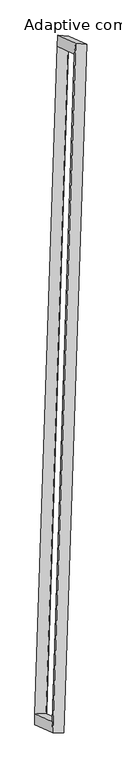
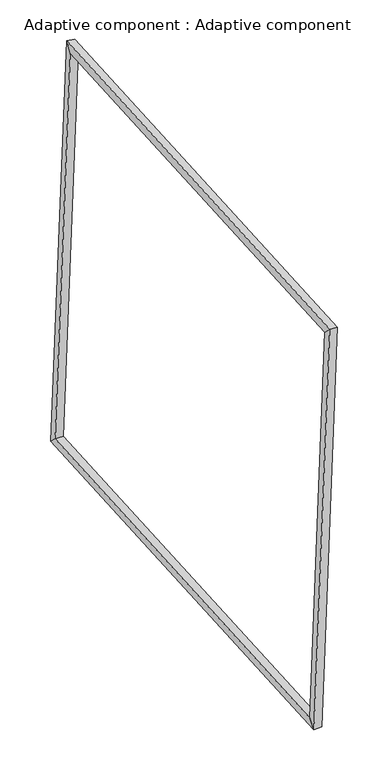
"""IFC4 building model written with IfcOpenShell, lengths in millimetres: proxy geometry, Adaptive component : Adaptive component."""

from ifc_helpers import new_model, si_unit, origin, place, context, project, spatial, faceted_brep, source, transform, mapped, element, save


def adaptive_component_adaptive_component_f8707263(model_context):
    return source(origin(), model_context, "Body", "Brep", [
        faceted_brep([(90.3369049, 1495.2326246, 3057.0965075), (154.9507537, 1489.5796526, 3051.5404015), (26.4269015, -2378.2634485, 3002.3473224), (-38.4243389, -2379.7546235, 3007.8125658), (97.9728871, 1559.0874571, 3122.6821483), (-35.0988393, -2445.6210085, 3071.7483501), (162.5867359, 1553.4344851, 3117.1260423), (29.752401, -2444.1298335, 3066.2831067), (-72.6526133, -2332.1726033, -362.721099), (-137.7142249, -2333.5659156, -364.4007569), (-138.20858, -2397.6553407, -430.1998857), (-73.1469685, -2396.2620283, -428.5202277), (55.8712389, 1535.6704978, -313.5280199), (-8.9529811, 1541.4213325, -315.1168152), (-5.1368535, 1607.0531249, -379.2660874), (59.6873664, 1601.3022902, -377.6772922)], [[[0, 1, 2, 3]], [[4, 0, 3, 5]], [[6, 4, 5, 7]], [[1, 6, 7, 2]], [[3, 2, 8, 9]], [[5, 3, 9, 10]], [[7, 5, 10, 11]], [[2, 7, 11, 8]], [[9, 8, 12, 13]], [[10, 9, 13, 14]], [[11, 10, 14, 15]], [[8, 11, 15, 12]], [[13, 12, 1, 0]], [[14, 13, 0, 4]], [[15, 14, 4, 6]], [[12, 15, 6, 1]]]),
    ])


if __name__ == "__main__":
    model = new_model("IFC4")
    model_context = context("Model", 3, world=origin())
    ifc_project = project(units=[si_unit("LENGTHUNIT", "METRE", prefix="MILLI")], contexts=[model_context])
    site = spatial("IfcSite", under=ifc_project)
    building = spatial("IfcBuilding", under=site)
    placement = place(None, origin())
    adaptive_component_adaptive_component_shape = adaptive_component_adaptive_component_f8707263(model_context)
    element("IfcBuildingElementProxy", 1, Name="Adaptive component : Adaptive component", ObjectType="Adaptive component : Adaptive component", at=placement, inside=building, context=model_context, shape_type="MappedRepresentation", body=[
        mapped(adaptive_component_adaptive_component_shape, transform((0.0, 0.0, 0.0), x_axis=(1.0, 0.0, 0.0), y_axis=(0.0, 1.0, 0.0), z_axis=(0.0, 0.0, 1.0))),
    ])
    save(model, "model.ifc")

# Revit data of these elements
# Type "Adaptive component : Adaptive component"
#   r [instance default] = 2063.125 mm
#   2r [instance default] = 4126.251 mm
#   Number [instance default] = 5
#   Default Elevation = 0
# Element 1 (IfcBuildingElementProxy, "Adaptive component : Adaptive component")
#   r = 2658.834 mm
#   2r = 5317.668 mm
#   Number = 26
